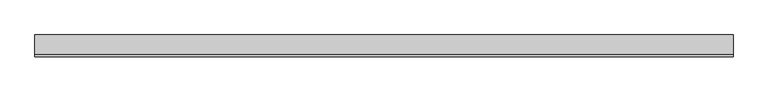
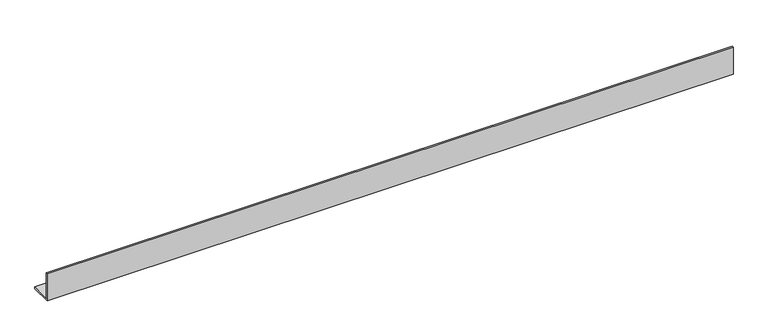
"""IFC4 building model written with IfcOpenShell, lengths in millimetres: proxy geometry, Generic Models 3:Generic Models 1:6:Generic Models 1:6 : Generic Models 3:Generic Models 1:300625:350611:Generic Models 1:6:Generic Models 1:6 : Generic Models 3:Generic Models 1:300625:350611 : Generic Models 3:Generic Models 1:6:Generic Models 1:6 : Generic Models 3:Generic Models 1:300625:350611:6 : Generic Models 3:Generic Models 1:6:Generic Models 1:6 : Generic Models 3:Generic Models 1:300625:350611:Generic Models 1:6:Generic Models 1:6 : Generic Models 3:Generic Models 1:300625:350611 : Generic Models 3:Generic Models 1:6:Generic Models 1:6 : Generic Models 3:Generic Models 1:300625:350611:301824."""

from ifc_helpers import new_model, si_unit, frame, origin, place, context, project, spatial, polyline, outline, extrude, source, transform, mapped, element, save


def generic_models_62598147(model_context):
    return source(origin(), model_context, "Body", "SweptSolid", [
        extrude(outline(polyline([(-579000.6913841, 0.0), (-579000.6913841, 101.6), (-578994.3413841, 101.6), (-578994.3413841, 6.35), (-578924.4913841, 6.35), (-578924.4913841, 0.0), (-579000.6913841, 0.0)])), frame((570452.6367239, 0.0, 0.0), z_axis=(1.0, 0.0, 0.0), x_axis=(0.0, 1.0, 0.0)), (0.0, 0.0, 1.0), 2438.4),
    ])


if __name__ == "__main__":
    model = new_model("IFC4")
    model_context = context("Model", 3, world=origin())
    ifc_project = project(units=[si_unit("LENGTHUNIT", "METRE", prefix="MILLI")], contexts=[model_context])
    site = spatial("IfcSite", under=ifc_project)
    building = spatial("IfcBuilding", under=site)
    placement = place(None, origin())
    generic_models_shape = generic_models_62598147(model_context)
    element("IfcBuildingElementProxy", 1, Name="Generic Models 3:Generic Models 1:6:Generic Models 1:6 : Generic Models 3:Generic Models 1:300625:350611:Generic Models 1:6:Generic Models 1:6 : Generic Models 3:Generic Models 1:300625:350611 : Generic Models 3:Generic Models 1:6:Generic Models 1:6 : Generic Models 3:Generic Models 1:300625:350611:6 : Generic Models 3:Generic Models 1:6:Generic Models 1:6 : Generic Models 3:Generic Models 1:300625:350611:Generic Models 1:6:Generic Models 1:6 : Generic Models 3:Generic Models 1:300625:350611 : Generic Models 3:Generic Models 1:6:Generic Models 1:6 : Generic Models 3:Generic Models 1:300625:350611:301824", ObjectType="Generic Models 3:Generic Models 1:6:Generic Models 1:6 : Generic Models 3:Generic Models 1:300625:350611:Generic Models 1:6:Generic Models 1:6 : Generic Models 3:Generic Models 1:300625:350611 : Generic Models 3:Generic Models 1:6:Generic Models 1:6 : Generic Models 3:Generic Models 1:300625:350611:6 : Generic Models 3:Generic Models 1:6:Generic Models 1:6 : Generic Models 3:Generic Models 1:300625:350611:Generic Models 1:6:Generic Models 1:6 : Generic Models 3:Generic Models 1:300625:350611 : Generic Models 3:Generic Models 1:6:Generic Models 1:6 : Generic Models 3:Generic Models 1:300625:350611:301824", at=placement, inside=building, context=model_context, shape_type="MappedRepresentation", body=[
        mapped(generic_models_shape, transform((0.0, 0.0, 0.0), x_axis=(1.0, 0.0, 0.0), y_axis=(0.0, 1.0, 0.0), z_axis=(0.0, 0.0, 1.0))),
    ])
    save(model, "model.ifc")

# Revit data of these elements
# Type "Generic Models 3:Generic Models 1:6:Generic Models 1:6 : Generic Models 3:Generic Models 1:300625:350611:Generic Models 1:6:Generic Models 1:6 : Generic Models 3:Generic Models 1:300625:350611 : Generic Models 3:Generic Models 1:6:Generic Models 1:6 : Generic Models 3:Generic Models 1:300625:350611:6 : Generic Models 3:Generic Models 1:6:Generic Models 1:6 : Generic Models 3:Generic Models 1:300625:350611:Generic Models 1:6:Generic Models 1:6 : Generic Models 3:Generic Models 1:300625:350611 : Generic Models 3:Generic Models 1:6:Generic Models 1:6 : Generic Models 3:Generic Models 1:300625:350611:301824"
#   NameOverride = "Generic Models 3:Generic Models 1:6:Generic Models 1:6 : Generic Models 3:Generic Models 1:300625:350611:Generic Models 1:6:Generic Models 1:6 : Generic Models 3:Generic Models 1:300625:350611 : Generic Models 3:Generic Models 1:6:Generic Models 1:6 : Generic Models 3:Generic Models 1:300625:350611:301824"
#   ObjectTypeOverride = "Generic Models 1:6:Generic Models 1:6 : Generic Models 3:Generic Models 1:300625:350611 : Generic Models 3:Generic Models 1:6:Generic Models 1:6 : Generic Models 3:Generic Models 1:300625:350611"
#   Reference = "Generic Models 1"
#   Tag = "301824"
